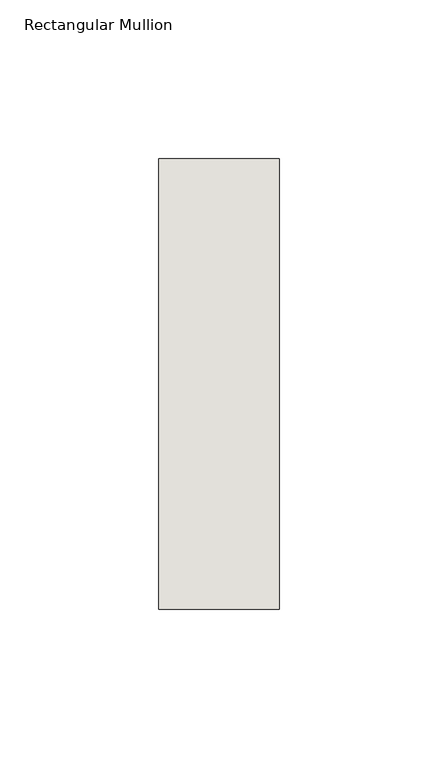
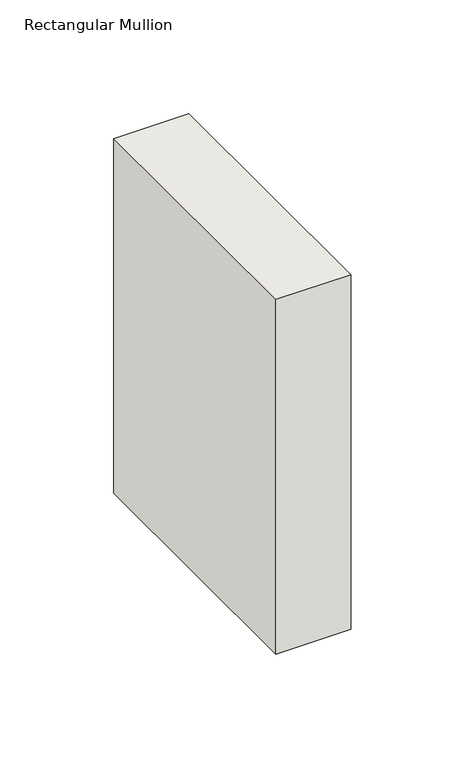
"""IFC4 building model written with IfcOpenShell, lengths in millimetres: wall geometry, Rectangular Mullion : NLRS_21_CWM_hsb-regel 38x142_gen_rsf."""

from ifc_helpers import new_model, si_unit, frame, origin, place, context, project, spatial, polyline, outline, extrude, source, transform, mapped, element, save


def rectangular_mullion_07180aef(model_context):
    return source(origin(), model_context, "Body", "SweptSolid", [
        extrude(outline(polyline([(-38.0, -71.0), (-38.0, 71.0), (0.0, 71.0), (0.0, -71.0), (-38.0, -71.0)])), frame((0.0, 0.0, -189.9999997), z_axis=(0.0, 0.0, 1.0), x_axis=(1.0, 0.0, 0.0)), (0.0, 0.0, 1.0), 189.9999997),
    ])


if __name__ == "__main__":
    model = new_model("IFC4")
    model_context = context("Model", 3, world=origin())
    ifc_project = project(units=[si_unit("LENGTHUNIT", "METRE", prefix="MILLI")], contexts=[model_context])
    site = spatial("IfcSite", under=ifc_project)
    building = spatial("IfcBuilding", under=site)
    placement = place(None, origin())
    rectangular_mullion_shape = rectangular_mullion_07180aef(model_context)
    element("IfcWall", 1, ObjectType="Rectangular Mullion : NLRS_21_CWM_hsb-regel 38x142_gen_rsf", at=placement, inside=building, context=model_context, shape_type="MappedRepresentation", body=[
        mapped(rectangular_mullion_shape, transform((0.0, 0.0, 0.0), x_axis=(1.0, 0.0, 0.0), y_axis=(0.0, 1.0, 0.0), z_axis=(0.0, 0.0, 1.0))),
    ])
    save(model, "model.ifc")

# Revit data of these elements
# Type "Rectangular Mullion : NLRS_21_CWM_hsb-regel 38x142_gen_rsf"
#   Type IfcGUID = "07M7mRoiH1CR8m_RSKIwpF"
#   Assembly Code = "21.10"
#   IfcExportAs = "IfcWall"
#   built-in parameter 1007322 = 0.465879 (stored number, unit not read)
#   built-in parameter 1007321 = 0.062336 (stored number, unit not read)
#   built-in parameter 1007320 = 0.062336 (stored number, unit not read)
# Element 1 (IfcWall, "Rectangular Mullion : NLRS_21_CWM_hsb-regel 38x142_gen_rsf")
#   Materials on its faces: "NLRS_i2_hout naaldhout vuren_gen_rsf"
# Materials
#   "NLRS_i2_hout naaldhout vuren_gen_rsf": class "I - Hout", colour RGB 234 199 147, transparency 0, Keynote = "i2", Manufacturer = "Revit Standards Foundation", URL = "www.revitstandards.org", Description = "hout vuren", Cost = 0
